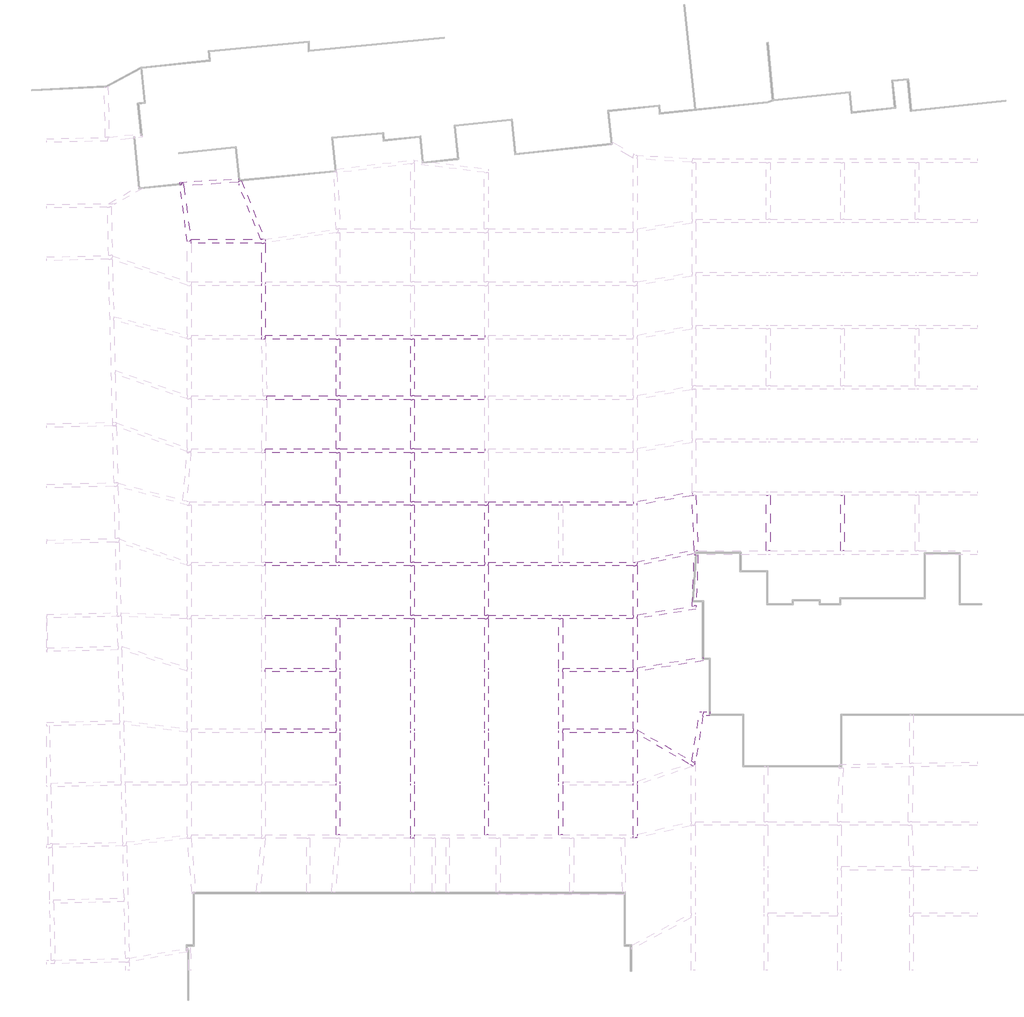
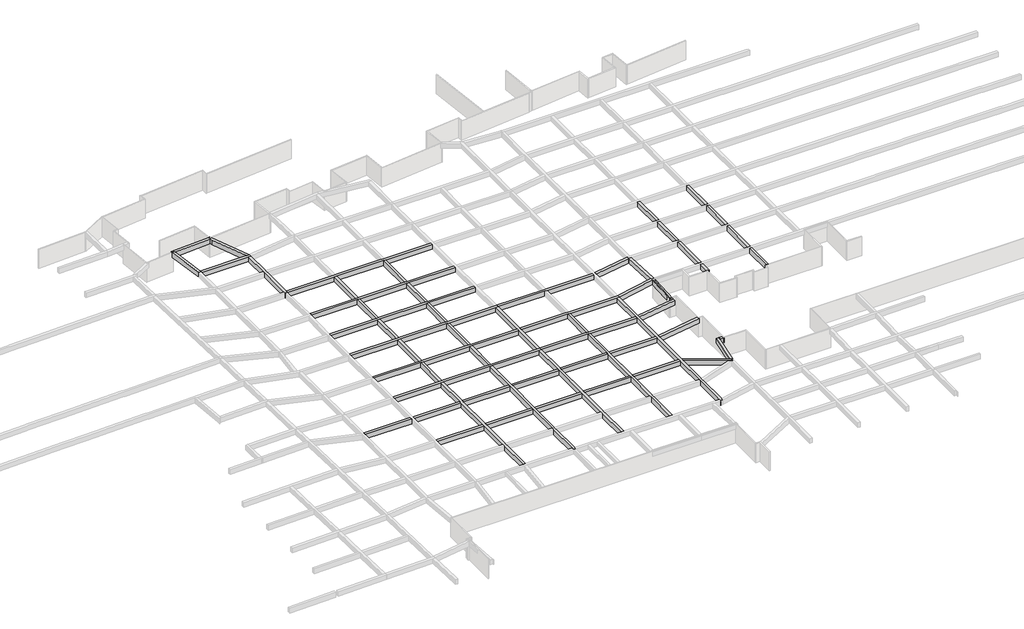
# One storey, part 18 of 20: 44 beams.
"""IFC4 building model written with IfcOpenShell, lengths in millimetres."""

from ifc_helpers import new_model, si_unit, frame, origin, place, context, project, spatial, polyline, outline, extrude, faceted_brep, element, save

model = new_model("IFC4")

# Units and contexts
model_context = context("Model", 3, world=origin())
ifc_project = project(units=[si_unit("LENGTHUNIT", "METRE", prefix="MILLI")], contexts=[model_context])

# Site, building, storey
site = spatial("IfcSite", under=ifc_project)
building = spatial("IfcBuilding", under=site)
storey = spatial("IfcBuildingStorey", under=building, Name="户型图", Elevation=0.0)

# Beams
placement = place(None, origin())
element("IfcBeam", 1, ObjectType="混凝土 - 矩形梁 : KL_beam", at=placement, inside=storey, context=model_context, shape_type="Brep", body=[
    faceted_brep([(54850.0, 183928.0776269, 3300.0), (54825.4500234, 184115.0, 3300.0), (54066.7931438, 189891.3779922, 3300.0), (54031.7451208, 190158.2319997, 3300.0), (53834.3182386, 190137.4815982, 3300.0), (53846.8616542, 190018.1389708, 3300.0), (53649.434772, 189997.3885693, 3300.0), (54450.0, 183901.9223731, 3300.0), (54450.0, 183901.9223731, 2500.0), (53649.434772, 189997.3885693, 2500.0), (54031.7451208, 190158.2319997, 2500.0), (54066.7931438, 189891.3779922, 2500.0), (54825.4500234, 184115.0, 2500.0), (54850.0, 183928.0776269, 2500.0), (53846.8616542, 190018.1389708, 2500.0), (53834.3182386, 190137.4815982, 2500.0)], [[[0, 1, 2, 3, 4, 5, 6, 7]], [[8, 7, 6, 9]], [[10, 11, 12, 13, 8, 9, 14, 15]], [[3, 2, 1, 0, 13, 12, 11, 10]], [[3, 10, 15, 4]], [[5, 14, 9, 6]], [[14, 5, 4, 15]], [[0, 7, 8, 13]]]),
])
element("IfcBeam", 2, ObjectType="混凝土 - 矩形梁 : KL_beam", at=placement, inside=storey, context=model_context, shape_type="Brep", body=[
    faceted_brep([(54825.4500234, 184115.0, 3300.0), (54850.0, 183928.0776269, 3300.0), (54850.0, 183715.0, 3300.0), (62450.0, 183715.0, 3300.0), (62850.0, 183715.0, 3300.0), (62850.0, 183741.1426524, 3300.0), (62850.0, 184115.0, 3300.0), (62636.0146376, 184115.0, 3300.0), (62354.8866617, 184115.0, 3300.0), (62850.0, 183715.0, 2500.0), (54850.0, 183715.0, 2500.0), (62450.0, 183715.0, 2500.0), (54850.0, 183928.0776269, 2500.0), (54825.4500234, 184115.0, 2500.0), (62354.8866617, 184115.0, 2500.0), (62636.0146376, 184115.0, 2500.0), (62850.0, 184115.0, 2500.0), (62850.0, 183741.1426524, 2500.0)], [[[0, 1, 2, 3, 4, 5, 6, 7, 8]], [[9, 4, 3, 2, 10, 11]], [[12, 13, 14, 15, 16, 17, 9, 11, 10]], [[13, 0, 8, 7, 6, 16, 15, 14]], [[1, 0, 13, 12]], [[2, 1, 12, 10]], [[6, 5, 4, 9, 17, 16]]]),
])
element("IfcBeam", 3, ObjectType="混凝土 - 矩形梁 : KL_beam", at=placement, inside=storey, context=model_context, shape_type="Brep", body=[
    faceted_brep([(62450.0, 173390.0, 3300.0), (62454.5621373, 173390.0, 3300.0), (62850.0, 173390.0, 3300.0), (62850.0, 173592.3073852, 3300.0), (62850.0, 173790.0, 3300.0), (62850.0, 179140.0, 3300.0), (62850.0, 179540.0, 3300.0), (62850.0, 183715.0, 3300.0), (62450.0, 183715.0, 3300.0), (62450.0, 179540.0, 3300.0), (62450.0, 179140.0, 3300.0), (62450.0, 173790.0, 3300.0), (62450.0, 173390.0, 2500.0), (62450.0, 183715.0, 2500.0), (62450.0, 179540.0, 2500.0), (62450.0, 179140.0, 2500.0), (62450.0, 173790.0, 2500.0), (62850.0, 173390.0, 2500.0), (62454.5621373, 173390.0, 2500.0), (62850.0, 183715.0, 2500.0), (62850.0, 179540.0, 2500.0), (62850.0, 179140.0, 2500.0), (62850.0, 173790.0, 2500.0), (62850.0, 173592.3073852, 2500.0)], [[[0, 1, 2, 3, 4, 5, 6, 7, 8, 9, 10, 11]], [[12, 0, 11, 10, 9, 8, 13, 14, 15, 16]], [[17, 18, 12, 16, 15, 14, 13, 19, 20, 21, 22, 23]], [[2, 17, 23, 22, 21, 20, 19, 7, 6, 5, 4, 3]], [[8, 7, 19, 13]], [[2, 1, 0, 12, 18, 17]]]),
])
element("IfcBeam", 4, ObjectType="混凝土 - 矩形梁 : KL_beam", at=placement, inside=storey, context=model_context, shape_type="Brep", body=[
    faceted_brep([(86850.0, 155490.0, 3300.0), (86850.0, 155890.0, 3300.0), (86450.0, 155890.0, 3300.0), (78871.1713568, 155890.0, 3300.0), (78471.1713568, 155890.0, 3300.0), (70871.1713568, 155890.0, 3300.0), (70471.1713568, 155890.0, 3300.0), (62850.0, 155890.0, 3300.0), (62850.0, 155490.0, 3300.0), (70471.1713568, 155490.0, 3300.0), (70871.1713568, 155490.0, 3300.0), (78471.1713568, 155490.0, 3300.0), (78871.1713568, 155490.0, 3300.0), (86450.0, 155490.0, 3300.0), (86850.0, 155490.0, 2500.0), (62850.0, 155490.0, 2500.0), (70471.1713568, 155490.0, 2500.0), (70871.1713568, 155490.0, 2500.0), (78471.1713568, 155490.0, 2500.0), (78871.1713568, 155490.0, 2500.0), (86450.0, 155490.0, 2500.0), (86850.0, 155890.0, 2500.0), (62850.0, 155890.0, 2500.0), (70471.1713568, 155890.0, 2500.0), (70871.1713568, 155890.0, 2500.0), (78471.1713568, 155890.0, 2500.0), (78871.1713568, 155890.0, 2500.0), (86450.0, 155890.0, 2500.0)], [[[0, 1, 2, 3, 4, 5, 6, 7, 8, 9, 10, 11, 12, 13]], [[14, 0, 13, 12, 11, 10, 9, 8, 15, 16, 17, 18, 19, 20]], [[21, 14, 20, 19, 18, 17, 16, 15, 22, 23, 24, 25, 26, 27]], [[1, 21, 27, 26, 25, 24, 23, 22, 7, 6, 5, 4, 3, 2]], [[8, 7, 22, 15]], [[1, 0, 14, 21]]]),
])
element("IfcBeam", 5, ObjectType="混凝土 - 矩形梁 : KL_beam", at=placement, inside=storey, context=model_context, shape_type="Brep", body=[
    faceted_brep([(62850.0, 149390.0, 3300.0), (62850.0, 148990.0, 3300.0), (70471.1713568, 148990.0, 3300.0), (70871.1713568, 148990.0, 3300.0), (78471.1713568, 148990.0, 3300.0), (78871.1713568, 148990.0, 3300.0), (86450.0, 148990.0, 3300.0), (86450.0, 149390.0, 3300.0), (78871.1713568, 149390.0, 3300.0), (78471.1713568, 149390.0, 3300.0), (70871.1713568, 149390.0, 3300.0), (70471.1713568, 149390.0, 3300.0), (62850.0, 148990.0, 2500.0), (70471.1713568, 148990.0, 2500.0), (70871.1713568, 148990.0, 2500.0), (78471.1713568, 148990.0, 2500.0), (78871.1713568, 148990.0, 2500.0), (86450.0, 148990.0, 2500.0), (62850.0, 149390.0, 2500.0), (70471.1713568, 149390.0, 2500.0), (70871.1713568, 149390.0, 2500.0), (78471.1713568, 149390.0, 2500.0), (78871.1713568, 149390.0, 2500.0), (86450.0, 149390.0, 2500.0)], [[[0, 1, 2, 3, 4, 5, 6, 7, 8, 9, 10, 11]], [[1, 12, 13, 14, 15, 16, 17, 6, 5, 4, 3, 2]], [[12, 18, 19, 20, 21, 22, 23, 17, 16, 15, 14, 13]], [[18, 0, 11, 10, 9, 8, 7, 23, 22, 21, 20, 19]], [[1, 0, 18, 12]], [[7, 6, 17, 23]]]),
])
element("IfcBeam", 6, ObjectType="混凝土 - 矩形梁 : KL_beam", at=placement, inside=storey, context=model_context, shape_type="Brep", body=[
    faceted_brep([(86850.0, 143290.0, 3300.0), (86850.0, 143690.0, 3300.0), (86450.0, 143690.0, 3300.0), (78871.1713568, 143690.0, 3300.0), (78471.1713568, 143690.0, 3300.0), (70871.1713568, 143690.0, 3300.0), (70471.1713568, 143690.0, 3300.0), (62850.0, 143690.0, 3300.0), (62850.0, 143290.0, 3300.0), (70471.1713568, 143290.0, 3300.0), (70871.1713568, 143290.0, 3300.0), (78471.1713568, 143290.0, 3300.0), (78871.1713568, 143290.0, 3300.0), (86450.0, 143290.0, 3300.0), (86850.0, 143290.0, 2500.0), (62850.0, 143290.0, 2500.0), (70471.1713568, 143290.0, 2500.0), (70871.1713568, 143290.0, 2500.0), (78471.1713568, 143290.0, 2500.0), (78871.1713568, 143290.0, 2500.0), (86450.0, 143290.0, 2500.0), (86850.0, 143690.0, 2500.0), (62850.0, 143690.0, 2500.0), (70471.1713568, 143690.0, 2500.0), (70871.1713568, 143690.0, 2500.0), (78471.1713568, 143690.0, 2500.0), (78871.1713568, 143690.0, 2500.0), (86450.0, 143690.0, 2500.0)], [[[0, 1, 2, 3, 4, 5, 6, 7, 8, 9, 10, 11, 12, 13]], [[14, 0, 13, 12, 11, 10, 9, 8, 15, 16, 17, 18, 19, 20]], [[21, 14, 20, 19, 18, 17, 16, 15, 22, 23, 24, 25, 26, 27]], [[1, 21, 27, 26, 25, 24, 23, 22, 7, 6, 5, 4, 3, 2]], [[8, 7, 22, 15]], [[1, 0, 14, 21]]]),
])
element("IfcBeam", 7, ObjectType="混凝土 - 矩形梁 : KL_beam", at=placement, inside=storey, context=model_context, shape_type="Brep", body=[
    faceted_brep([(62855.332398, 161590.0, 3300.0), (62850.0, 161387.3688765, 3300.0), (62850.0, 161190.0, 3300.0), (70471.1713568, 161190.0, 3300.0), (70871.1713568, 161190.0, 3300.0), (78471.1713568, 161190.0, 3300.0), (78871.1713568, 161190.0, 3300.0), (86450.0, 161190.0, 3300.0), (86450.0, 161590.0, 3300.0), (78871.1713568, 161590.0, 3300.0), (78471.1713568, 161590.0, 3300.0), (70871.1713568, 161590.0, 3300.0), (70471.1713568, 161590.0, 3300.0), (62850.0, 161190.0, 2500.0), (70471.1713568, 161190.0, 2500.0), (70871.1713568, 161190.0, 2500.0), (78471.1713568, 161190.0, 2500.0), (78871.1713568, 161190.0, 2500.0), (86450.0, 161190.0, 2500.0), (62850.0, 161387.3688765, 2500.0), (62855.332398, 161590.0, 2500.0), (70471.1713568, 161590.0, 2500.0), (70871.1713568, 161590.0, 2500.0), (78471.1713568, 161590.0, 2500.0), (78871.1713568, 161590.0, 2500.0), (86450.0, 161590.0, 2500.0)], [[[0, 1, 2, 3, 4, 5, 6, 7, 8, 9, 10, 11, 12]], [[2, 13, 14, 15, 16, 17, 18, 7, 6, 5, 4, 3]], [[19, 20, 21, 22, 23, 24, 25, 18, 17, 16, 15, 14, 13]], [[20, 0, 12, 11, 10, 9, 8, 25, 24, 23, 22, 21]], [[0, 20, 19, 1]], [[2, 1, 19, 13]], [[8, 7, 18, 25]]]),
])
element("IfcBeam", 8, ObjectType="混凝土 - 矩形梁 : KL_beam", at=placement, inside=storey, context=model_context, shape_type="Brep", body=[
    faceted_brep([(63000.0607194, 167089.6762125, 3300.0), (63004.668632, 166890.0, 3300.0), (70471.1713568, 166890.0, 3300.0), (70871.1713568, 166890.0, 3300.0), (78471.1713568, 166890.0, 3300.0), (78871.1713568, 166890.0, 3300.0), (86450.0, 166890.0, 3300.0), (86450.0, 167290.0, 3300.0), (78866.5603873, 167290.0, 3300.0), (78466.5603873, 167290.0, 3300.0), (70871.1713568, 167290.0, 3300.0), (70471.1713568, 167290.0, 3300.0), (63005.332398, 167290.0, 3300.0), (63004.668632, 166890.0, 2500.0), (70471.1713568, 166890.0, 2500.0), (70871.1713568, 166890.0, 2500.0), (78471.1713568, 166890.0, 2500.0), (78871.1713568, 166890.0, 2500.0), (86450.0, 166890.0, 2500.0), (63000.0607194, 167089.6762125, 2500.0), (63005.332398, 167290.0, 2500.0), (70471.1713568, 167290.0, 2500.0), (70871.1713568, 167290.0, 2500.0), (78466.5603873, 167290.0, 2500.0), (78866.5603873, 167290.0, 2500.0), (86450.0, 167290.0, 2500.0)], [[[0, 1, 2, 3, 4, 5, 6, 7, 8, 9, 10, 11, 12]], [[1, 13, 14, 15, 16, 17, 18, 6, 5, 4, 3, 2]], [[13, 19, 20, 21, 22, 23, 24, 25, 18, 17, 16, 15, 14]], [[20, 12, 11, 10, 9, 8, 7, 25, 24, 23, 22, 21]], [[13, 1, 0, 19]], [[0, 12, 20, 19]], [[7, 6, 18, 25]]]),
])
element("IfcBeam", 9, ObjectType="混凝土 - 矩形梁 : KL_beam", at=placement, inside=storey, context=model_context, shape_type="Brep", body=[
    faceted_brep([(62850.0, 173790.0, 3300.0), (62850.0, 173592.3073852, 3300.0), (62854.668632, 173390.0, 3300.0), (70471.1713568, 173390.0, 3300.0), (70871.1713568, 173390.0, 3300.0), (78466.5603873, 173390.0, 3300.0), (78866.5603873, 173390.0, 3300.0), (86450.0, 173390.0, 3300.0), (86450.0, 173790.0, 3300.0), (78866.5603873, 173790.0, 3300.0), (78466.5603873, 173790.0, 3300.0), (70871.1713568, 173790.0, 3300.0), (70471.1713568, 173790.0, 3300.0), (62854.668632, 173390.0, 2500.0), (70471.1713568, 173390.0, 2500.0), (70871.1713568, 173390.0, 2500.0), (78466.5603873, 173390.0, 2500.0), (78866.5603873, 173390.0, 2500.0), (86450.0, 173390.0, 2500.0), (62850.0, 173592.3073852, 2500.0), (62850.0, 173790.0, 2500.0), (70471.1713568, 173790.0, 2500.0), (70871.1713568, 173790.0, 2500.0), (78466.5603873, 173790.0, 2500.0), (78866.5603873, 173790.0, 2500.0), (86450.0, 173790.0, 2500.0)], [[[0, 1, 2, 3, 4, 5, 6, 7, 8, 9, 10, 11, 12]], [[2, 13, 14, 15, 16, 17, 18, 7, 6, 5, 4, 3]], [[19, 20, 21, 22, 23, 24, 25, 18, 17, 16, 15, 14, 13]], [[20, 0, 12, 11, 10, 9, 8, 25, 24, 23, 22, 21]], [[0, 20, 19, 1]], [[2, 1, 19, 13]], [[8, 7, 18, 25]]]),
])
element("IfcBeam", 10, ObjectType="混凝土 - 矩形梁 : KL_beam", at=placement, inside=storey, context=model_context, shape_type="Brep", body=[
    faceted_brep([(60034.1132037, 189932.4884269, 3300.0), (60034.1132037, 189932.4884269, 2500.0), (62354.8866617, 184115.0, 2500.0), (62354.8866617, 184115.0, 3300.0), (59999.9831265, 190257.2144199, 3300.0), (59985.5481909, 190394.5536585, 3300.0), (59985.5481909, 190394.5536585, 2500.0), (59999.9831265, 190257.2144199, 2500.0), (60269.4868427, 190421.9993923, 3300.0), (60269.4868427, 190421.9993923, 2500.0), (62450.0, 184115.0, 2500.0), (62636.0146376, 184115.0, 2500.0), (62636.0146376, 184115.0, 3300.0), (62450.0, 184115.0, 3300.0), (62777.6028574, 184134.8989266, 3300.0), (62777.6028574, 184134.8989266, 2500.0)], [[[0, 1, 2, 3]], [[1, 0, 4, 5, 6, 7]], [[5, 8, 9, 6]], [[3, 2, 10, 11, 12, 13]], [[5, 4, 0, 3, 13, 12, 14, 8]], [[1, 7, 6, 9, 15, 11, 10, 2]], [[9, 8, 14, 15]], [[12, 11, 15, 14]]]),
])
element("IfcBeam", 11, ObjectType="混凝土 - 矩形梁 : KL_beam", at=placement, inside=storey, context=model_context, shape_type="Brep", body=[
    faceted_brep([(60171.1392883, 190668.5274444, 3300.0), (60078.0168735, 190662.7855801, 3300.0), (60092.4518091, 190525.4463415, 3300.0), (60223.1777857, 190538.0824174, 3300.0), (60078.0168735, 190662.7855801, 2500.0), (60171.1392883, 190668.5274444, 2500.0), (60223.1777857, 190538.0824174, 2500.0), (60092.4518091, 190525.4463415, 2500.0)], [[[0, 1, 2, 3]], [[4, 5, 6, 7]], [[0, 5, 4, 1]], [[5, 0, 3, 6]], [[2, 1, 4, 7]], [[3, 2, 7, 6]]]),
    faceted_brep([(59999.9831265, 190257.2144199, 2500.0), (59999.9831265, 190257.2144199, 3300.0), (54066.7931438, 189891.3779922, 3300.0), (54066.7931438, 189891.3779922, 2500.0), (53614.386749, 190264.2425768, 3300.0), (53614.386749, 190264.2425768, 2500.0), (53633.8032011, 190116.4066185, 2500.0), (53633.8032011, 190116.4066185, 3300.0), (59958.1328072, 190655.3936108, 2500.0), (59958.1328072, 190655.3936108, 3300.0), (59985.5481909, 190394.5536585, 3300.0), (59985.5481909, 190394.5536585, 2500.0), (53834.3182386, 190137.4815982, 2500.0), (54031.7451208, 190158.2319997, 2500.0), (54031.7451208, 190158.2319997, 3300.0), (53834.3182386, 190137.4815982, 3300.0)], [[[0, 1, 2, 3]], [[4, 5, 6, 7]], [[8, 9, 10, 1, 0, 11]], [[5, 4, 9, 8]], [[7, 6, 12, 13, 14, 15]], [[9, 4, 7, 15, 14, 2, 1, 10]], [[5, 8, 11, 0, 3, 13, 12, 6]], [[14, 13, 3, 2]]]),
])
element("IfcBeam", 12, ObjectType="混凝土 - 矩形梁 : KL_beam", at=placement, inside=storey, context=model_context, shape_type="SweptSolid", body=[
    extrude(outline(polyline([(70871.1713568, 167290.0), (70471.1713568, 167290.0), (70471.1713568, 173390.0), (70871.1713568, 173390.0), (70871.1713568, 167290.0)])), frame((0.0, 0.0, 2500.0), z_axis=(0.0, 0.0, 1.0), x_axis=(1.0, 0.0, 0.0)), (0.0, 0.0, 1.0), 800.0),
])
element("IfcBeam", 13, ObjectType="混凝土 - 矩形梁 : KL_beam", at=placement, inside=storey, context=model_context, shape_type="SweptSolid", body=[
    extrude(outline(polyline([(70871.1713568, 161590.0), (70471.1713568, 161590.0), (70471.1713568, 166890.0), (70871.1713568, 166890.0), (70871.1713568, 161590.0)])), frame((0.0, 0.0, 2500.0), z_axis=(0.0, 0.0, 1.0), x_axis=(1.0, 0.0, 0.0)), (0.0, 0.0, 1.0), 800.0),
])
element("IfcBeam", 14, ObjectType="混凝土 - 矩形梁 : KL_beam", at=placement, inside=storey, context=model_context, shape_type="SweptSolid", body=[
    extrude(outline(polyline([(70871.1713568, 155890.0), (70471.1713568, 155890.0), (70471.1713568, 161190.0), (70871.1713568, 161190.0), (70871.1713568, 155890.0)])), frame((0.0, 0.0, 2500.0), z_axis=(0.0, 0.0, 1.0), x_axis=(1.0, 0.0, 0.0)), (0.0, 0.0, 1.0), 800.0),
])
element("IfcBeam", 15, ObjectType="混凝土 - 矩形梁 : KL_beam", at=placement, inside=storey, context=model_context, shape_type="SweptSolid", body=[
    extrude(outline(polyline([(70471.1713568, 155490.0), (70871.1713568, 155490.0), (70871.1713568, 149390.0), (70471.1713568, 149390.0), (70471.1713568, 155490.0)])), frame((0.0, 0.0, 2500.0), z_axis=(0.0, 0.0, 1.0), x_axis=(1.0, 0.0, 0.0)), (0.0, 0.0, 1.0), 800.0),
    extrude(outline(polyline([(70871.1713568, 143690.0), (70471.1713568, 143690.0), (70471.1713568, 148990.0), (70871.1713568, 148990.0), (70871.1713568, 143690.0)])), frame((0.0, 0.0, 2500.0), z_axis=(0.0, 0.0, 1.0), x_axis=(1.0, 0.0, 0.0)), (0.0, 0.0, 1.0), 800.0),
])
element("IfcBeam", 16, ObjectType="混凝土 - 矩形梁 : KL_beam", at=placement, inside=storey, context=model_context, shape_type="SweptSolid", body=[
    extrude(outline(polyline([(78471.1713568, 148990.0), (78871.1713568, 148990.0), (78871.1713568, 143690.0), (78471.1713568, 143690.0), (78471.1713568, 148990.0)])), frame((0.0, 0.0, 2500.0), z_axis=(0.0, 0.0, 1.0), x_axis=(1.0, 0.0, 0.0)), (0.0, 0.0, 1.0), 800.0),
])
element("IfcBeam", 17, ObjectType="混凝土 - 矩形梁 : KL_beam", at=placement, inside=storey, context=model_context, shape_type="SweptSolid", body=[
    extrude(outline(polyline([(78471.1713568, 155490.0), (78871.1713568, 155490.0), (78871.1713568, 149390.0), (78471.1713568, 149390.0), (78471.1713568, 155490.0)])), frame((0.0, 0.0, 2500.0), z_axis=(0.0, 0.0, 1.0), x_axis=(1.0, 0.0, 0.0)), (0.0, 0.0, 1.0), 800.0),
])
element("IfcBeam", 18, ObjectType="混凝土 - 矩形梁 : KL_beam", at=placement, inside=storey, context=model_context, shape_type="SweptSolid", body=[
    extrude(outline(polyline([(78871.1713568, 155890.0), (78471.1713568, 155890.0), (78471.1713568, 161190.0), (78871.1713568, 161190.0), (78871.1713568, 155890.0)])), frame((0.0, 0.0, 2500.0), z_axis=(0.0, 0.0, 1.0), x_axis=(1.0, 0.0, 0.0)), (0.0, 0.0, 1.0), 800.0),
])
element("IfcBeam", 19, ObjectType="混凝土 - 矩形梁 : KL_beam", at=placement, inside=storey, context=model_context, shape_type="SweptSolid", body=[
    extrude(outline(polyline([(78871.1713568, 161590.0), (78471.1713568, 161590.0), (78471.1713568, 166890.0), (78871.1713568, 166890.0), (78871.1713568, 161590.0)])), frame((0.0, 0.0, 2500.0), z_axis=(0.0, 0.0, 1.0), x_axis=(1.0, 0.0, 0.0)), (0.0, 0.0, 1.0), 800.0),
])
element("IfcBeam", 20, ObjectType="混凝土 - 矩形梁 : KL_beam", at=placement, inside=storey, context=model_context, shape_type="SweptSolid", body=[
    extrude(outline(polyline([(78866.5603873, 167290.0), (78466.5603873, 167290.0), (78466.5603873, 173390.0), (78866.5603873, 173390.0), (78866.5603873, 167290.0)])), frame((0.0, 0.0, 2500.0), z_axis=(0.0, 0.0, 1.0), x_axis=(1.0, 0.0, 0.0)), (0.0, 0.0, 1.0), 800.0),
])
element("IfcBeam", 21, ObjectType="混凝土 - 矩形梁 : KL_beam", at=placement, inside=storey, context=model_context, shape_type="Brep", body=[
    faceted_brep([(86850.0, 155490.0, 3300.0), (86450.0, 155490.0, 3300.0), (86450.0, 149390.0, 3300.0), (86450.0, 148990.0, 3300.0), (86450.0, 143690.0, 3300.0), (86850.0, 143690.0, 3300.0), (86850.0, 148990.0, 3300.0), (86850.0, 149390.0, 3300.0), (86450.0, 155490.0, 2500.0), (86450.0, 149390.0, 2500.0), (86450.0, 148990.0, 2500.0), (86450.0, 143690.0, 2500.0), (86850.0, 155490.0, 2500.0), (86850.0, 149390.0, 2500.0), (86850.0, 148990.0, 2500.0), (86850.0, 143690.0, 2500.0)], [[[0, 1, 2, 3, 4, 5, 6, 7]], [[1, 8, 9, 10, 11, 4, 3, 2]], [[8, 12, 13, 14, 15, 11, 10, 9]], [[12, 0, 7, 6, 5, 15, 14, 13]], [[1, 0, 12, 8]], [[5, 4, 11, 15]]]),
])
element("IfcBeam", 22, ObjectType="混凝土 - 矩形梁 : KL_beam", at=placement, inside=storey, context=model_context, shape_type="Brep", body=[
    faceted_brep([(86850.0, 155890.0, 3300.0), (86850.0, 155490.0, 3300.0), (94423.4648002, 155490.0, 3300.0), (94823.4648002, 155490.0, 3300.0), (102450.0, 155490.0, 3300.0), (102450.0, 155890.0, 3300.0), (94823.4648002, 155890.0, 3300.0), (94423.4648002, 155890.0, 3300.0), (86850.0, 155490.0, 2500.0), (94423.4648002, 155490.0, 2500.0), (94823.4648002, 155490.0, 2500.0), (102450.0, 155490.0, 2500.0), (86850.0, 155890.0, 2500.0), (94423.4648002, 155890.0, 2500.0), (94823.4648002, 155890.0, 2500.0), (102450.0, 155890.0, 2500.0)], [[[0, 1, 2, 3, 4, 5, 6, 7]], [[1, 8, 9, 10, 11, 4, 3, 2]], [[8, 12, 13, 14, 15, 11, 10, 9]], [[12, 0, 7, 6, 5, 15, 14, 13]], [[1, 0, 12, 8]], [[5, 4, 11, 15]]]),
])
element("IfcBeam", 23, ObjectType="混凝土 - 矩形梁 : KL_beam", at=placement, inside=storey, context=model_context, shape_type="Brep", body=[
    faceted_brep([(102850.0, 148990.0, 3300.0), (102850.0, 149026.9931985, 3300.0), (102850.0, 149390.0, 3300.0), (102450.0, 149390.0, 3300.0), (94823.4648002, 149390.0, 3300.0), (94423.4648002, 149390.0, 3300.0), (86850.0, 149390.0, 3300.0), (86850.0, 148990.0, 3300.0), (94423.4648002, 148990.0, 3300.0), (94823.4648002, 148990.0, 3300.0), (102450.0, 148990.0, 3300.0), (102850.0, 148990.0, 2500.0), (86850.0, 148990.0, 2500.0), (94423.4648002, 148990.0, 2500.0), (94823.4648002, 148990.0, 2500.0), (102450.0, 148990.0, 2500.0), (102850.0, 149390.0, 2500.0), (102850.0, 149026.9931985, 2500.0), (86850.0, 149390.0, 2500.0), (94423.4648002, 149390.0, 2500.0), (94823.4648002, 149390.0, 2500.0), (102450.0, 149390.0, 2500.0)], [[[0, 1, 2, 3, 4, 5, 6, 7, 8, 9, 10]], [[11, 0, 10, 9, 8, 7, 12, 13, 14, 15]], [[16, 17, 11, 15, 14, 13, 12, 18, 19, 20, 21]], [[2, 16, 21, 20, 19, 18, 6, 5, 4, 3]], [[7, 6, 18, 12]], [[2, 1, 0, 11, 17, 16]]]),
])
element("IfcBeam", 24, ObjectType="混凝土 - 矩形梁 : KL_beam", at=placement, inside=storey, context=model_context, shape_type="Brep", body=[
    faceted_brep([(86850.0, 143690.0, 3300.0), (86850.0, 143290.0, 3300.0), (94423.4648002, 143290.0, 3300.0), (94823.4648002, 143290.0, 3300.0), (102450.0, 143290.0, 3300.0), (102450.0, 143690.0, 3300.0), (94823.4648002, 143690.0, 3300.0), (94423.4648002, 143690.0, 3300.0), (86850.0, 143290.0, 2500.0), (94423.4648002, 143290.0, 2500.0), (94823.4648002, 143290.0, 2500.0), (102450.0, 143290.0, 2500.0), (86850.0, 143690.0, 2500.0), (94423.4648002, 143690.0, 2500.0), (94823.4648002, 143690.0, 2500.0), (102450.0, 143690.0, 2500.0)], [[[0, 1, 2, 3, 4, 5, 6, 7]], [[1, 8, 9, 10, 11, 4, 3, 2]], [[8, 12, 13, 14, 15, 11, 10, 9]], [[12, 0, 7, 6, 5, 15, 14, 13]], [[1, 0, 12, 8]], [[5, 4, 11, 15]]]),
])
element("IfcBeam", 25, ObjectType="混凝土 - 矩形梁 : KL_beam", at=placement, inside=storey, context=model_context, shape_type="Brep", body=[
    faceted_brep([(102850.0, 119729.9007984, 3300.0), (102850.0, 120139.8450935, 3300.0), (102850.0, 125421.4252388, 3300.0), (102850.0, 125843.4152433, 3300.0), (102850.0, 130914.5836602, 3300.0), (102850.0, 131376.4638755, 3300.0), (102850.0, 137632.1126937, 3300.0), (102850.0, 138037.3913563, 3300.0), (102850.0, 143319.1838629, 3300.0), (102850.0, 143724.1699132, 3300.0), (102850.0, 148990.0, 3300.0), (102450.0, 148990.0, 3300.0), (102450.0, 143690.0, 3300.0), (102450.0, 143290.0, 3300.0), (102450.0, 138002.152967, 3300.0), (102450.0, 137602.152967, 3300.0), (102450.0, 131460.9938217, 3300.0), (102450.0, 131060.9938217, 3300.0), (102450.0, 125765.1975441, 3300.0), (102450.0, 125365.1975441, 3300.0), (102450.0, 120090.0, 3300.0), (102450.0, 119729.9007984, 3300.0), (102450.0, 148990.0, 2500.0), (102450.0, 143690.0, 2500.0), (102450.0, 143290.0, 2500.0), (102450.0, 138002.152967, 2500.0), (102450.0, 137602.152967, 2500.0), (102450.0, 131460.9938217, 2500.0), (102450.0, 131060.9938217, 2500.0), (102450.0, 125765.1975441, 2500.0), (102450.0, 125365.1975441, 2500.0), (102450.0, 120090.0, 2500.0), (102450.0, 119729.9007984, 2500.0), (102850.0, 148990.0, 2500.0), (102850.0, 143724.1699132, 2500.0), (102850.0, 143319.1838629, 2500.0), (102850.0, 138037.3913563, 2500.0), (102850.0, 137632.1126937, 2500.0), (102850.0, 131376.4638755, 2500.0), (102850.0, 130914.5836602, 2500.0), (102850.0, 125843.4152433, 2500.0), (102850.0, 125421.4252388, 2500.0), (102850.0, 120139.8450935, 2500.0), (102850.0, 119729.9007984, 2500.0)], [[[0, 1, 2, 3, 4, 5, 6, 7, 8, 9, 10, 11, 12, 13, 14, 15, 16, 17, 18, 19, 20, 21]], [[21, 20, 19, 18, 17, 16, 15, 14, 13, 12, 11, 22, 23, 24, 25, 26, 27, 28, 29, 30, 31, 32]], [[32, 31, 30, 29, 28, 27, 26, 25, 24, 23, 22, 33, 34, 35, 36, 37, 38, 39, 40, 41, 42, 43]], [[10, 9, 8, 7, 6, 5, 4, 3, 2, 1, 0, 43, 42, 41, 40, 39, 38, 37, 36, 35, 34, 33]], [[11, 10, 33, 22]], [[0, 21, 32, 43]]]),
])
element("IfcBeam", 26, ObjectType="混凝土 - 矩形梁 : KL_beam", at=placement, inside=storey, context=model_context, shape_type="Brep", body=[
    faceted_brep([(94823.4648002, 148990.0, 3300.0), (94423.4648002, 148990.0, 3300.0), (94423.4648002, 143690.0, 3300.0), (94823.4648002, 143690.0, 3300.0), (94423.4648002, 148990.0, 2500.0), (94423.4648002, 143690.0, 2500.0), (94823.4648002, 148990.0, 2500.0), (94823.4648002, 143690.0, 2500.0)], [[[0, 1, 2, 3]], [[1, 4, 5, 2]], [[4, 6, 7, 5]], [[6, 0, 3, 7]], [[1, 0, 6, 4]], [[3, 2, 5, 7]]]),
    faceted_brep([(94423.4648002, 143290.0, 3300.0), (94823.4648002, 143290.0, 3300.0), (94823.4648002, 143290.0, 2500.0), (94423.4648002, 143290.0, 2500.0), (94423.4648002, 138002.152967, 3300.0), (94423.4648002, 137602.152967, 3300.0), (94423.4648002, 131460.9938217, 3300.0), (94423.4648002, 131060.9938217, 3300.0), (94423.4648002, 125765.1975441, 3300.0), (94423.4648002, 125365.1975441, 3300.0), (94423.4648002, 120090.0, 3300.0), (94823.4648002, 120090.0, 3300.0), (94823.4648002, 125365.1975441, 3300.0), (94823.4648002, 125765.1975441, 3300.0), (94823.4648002, 131060.9938217, 3300.0), (94823.4648002, 131460.9938217, 3300.0), (94823.4648002, 137602.152967, 3300.0), (94823.4648002, 138002.152967, 3300.0), (94423.4648002, 138002.152967, 2500.0), (94423.4648002, 137602.152967, 2500.0), (94423.4648002, 131460.9938217, 2500.0), (94423.4648002, 131060.9938217, 2500.0), (94423.4648002, 125765.1975441, 2500.0), (94423.4648002, 125365.1975441, 2500.0), (94423.4648002, 120090.0, 2500.0), (94823.4648002, 138002.152967, 2500.0), (94823.4648002, 137602.152967, 2500.0), (94823.4648002, 131460.9938217, 2500.0), (94823.4648002, 131060.9938217, 2500.0), (94823.4648002, 125765.1975441, 2500.0), (94823.4648002, 125365.1975441, 2500.0), (94823.4648002, 120090.0, 2500.0)], [[[0, 1, 2, 3]], [[1, 0, 4, 5, 6, 7, 8, 9, 10, 11, 12, 13, 14, 15, 16, 17]], [[0, 3, 18, 19, 20, 21, 22, 23, 24, 10, 9, 8, 7, 6, 5, 4]], [[3, 2, 25, 26, 27, 28, 29, 30, 31, 24, 23, 22, 21, 20, 19, 18]], [[2, 1, 17, 16, 15, 14, 13, 12, 11, 31, 30, 29, 28, 27, 26, 25]], [[11, 10, 24, 31]]]),
])
element("IfcBeam", 27, ObjectType="混凝土 - 矩形梁 : KL_beam", at=placement, inside=storey, context=model_context, shape_type="Brep", body=[
    faceted_brep([(86850.0, 143290.0, 3300.0), (86450.0, 143290.0, 3300.0), (86450.0, 138002.152967, 3300.0), (86450.0, 137602.152967, 3300.0), (86450.0, 131460.9938217, 3300.0), (86450.0, 131060.9938217, 3300.0), (86450.0, 125765.1975441, 3300.0), (86450.0, 125365.1975441, 3300.0), (86450.0, 120090.0, 3300.0), (86850.0, 120090.0, 3300.0), (86850.0, 125365.1975441, 3300.0), (86850.0, 125765.1975441, 3300.0), (86850.0, 131060.9938217, 3300.0), (86850.0, 131460.9938217, 3300.0), (86850.0, 137602.152967, 3300.0), (86850.0, 138002.152967, 3300.0), (86450.0, 143290.0, 2500.0), (86450.0, 138002.152967, 2500.0), (86450.0, 137602.152967, 2500.0), (86450.0, 131460.9938217, 2500.0), (86450.0, 131060.9938217, 2500.0), (86450.0, 125765.1975441, 2500.0), (86450.0, 125365.1975441, 2500.0), (86450.0, 120090.0, 2500.0), (86850.0, 143290.0, 2500.0), (86850.0, 138002.152967, 2500.0), (86850.0, 137602.152967, 2500.0), (86850.0, 131460.9938217, 2500.0), (86850.0, 131060.9938217, 2500.0), (86850.0, 125765.1975441, 2500.0), (86850.0, 125365.1975441, 2500.0), (86850.0, 120090.0, 2500.0)], [[[0, 1, 2, 3, 4, 5, 6, 7, 8, 9, 10, 11, 12, 13, 14, 15]], [[1, 16, 17, 18, 19, 20, 21, 22, 23, 8, 7, 6, 5, 4, 3, 2]], [[16, 24, 25, 26, 27, 28, 29, 30, 31, 23, 22, 21, 20, 19, 18, 17]], [[24, 0, 15, 14, 13, 12, 11, 10, 9, 31, 30, 29, 28, 27, 26, 25]], [[1, 0, 24, 16]], [[9, 8, 23, 31]]]),
])
element("IfcBeam", 28, ObjectType="混凝土 - 矩形梁 : KL_beam", at=placement, inside=storey, context=model_context, shape_type="Brep", body=[
    faceted_brep([(78471.1713568, 119690.0, 3300.0), (78871.1713568, 119690.0, 3300.0), (78871.1713568, 120090.0, 3300.0), (78871.1713568, 125365.1975441, 3300.0), (78871.1713568, 125765.1975441, 3300.0), (78871.1713568, 131060.9938217, 3300.0), (78871.1713568, 131460.9938217, 3300.0), (78871.1713568, 137602.152967, 3300.0), (78871.1713568, 138002.152967, 3300.0), (78871.1713568, 143290.0, 3300.0), (78471.1713568, 143290.0, 3300.0), (78471.1713568, 138002.152967, 3300.0), (78471.1713568, 137602.152967, 3300.0), (78471.1713568, 131460.9938217, 3300.0), (78471.1713568, 131060.9938217, 3300.0), (78471.1713568, 125765.1975441, 3300.0), (78471.1713568, 125365.1975441, 3300.0), (78471.1713568, 120090.0, 3300.0), (78471.1713568, 119690.0, 2500.0), (78471.1713568, 143290.0, 2500.0), (78471.1713568, 138002.152967, 2500.0), (78471.1713568, 137602.152967, 2500.0), (78471.1713568, 131460.9938217, 2500.0), (78471.1713568, 131060.9938217, 2500.0), (78471.1713568, 125765.1975441, 2500.0), (78471.1713568, 125365.1975441, 2500.0), (78471.1713568, 120090.0, 2500.0), (78871.1713568, 119690.0, 2500.0), (78871.1713568, 143290.0, 2500.0), (78871.1713568, 138002.152967, 2500.0), (78871.1713568, 137602.152967, 2500.0), (78871.1713568, 131460.9938217, 2500.0), (78871.1713568, 131060.9938217, 2500.0), (78871.1713568, 125765.1975441, 2500.0), (78871.1713568, 125365.1975441, 2500.0), (78871.1713568, 120090.0, 2500.0)], [[[0, 1, 2, 3, 4, 5, 6, 7, 8, 9, 10, 11, 12, 13, 14, 15, 16, 17]], [[18, 0, 17, 16, 15, 14, 13, 12, 11, 10, 19, 20, 21, 22, 23, 24, 25, 26]], [[27, 18, 26, 25, 24, 23, 22, 21, 20, 19, 28, 29, 30, 31, 32, 33, 34, 35]], [[1, 27, 35, 34, 33, 32, 31, 30, 29, 28, 9, 8, 7, 6, 5, 4, 3, 2]], [[10, 9, 28, 19]], [[1, 0, 18, 27]]]),
])
element("IfcBeam", 29, ObjectType="混凝土 - 矩形梁 : KL_beam", at=placement, inside=storey, context=model_context, shape_type="Brep", body=[
    faceted_brep([(70871.1713568, 143290.0, 3300.0), (70471.1713568, 143290.0, 3300.0), (70471.1713568, 138002.152967, 3300.0), (70471.1713568, 137602.152967, 3300.0), (70471.1713568, 131460.9938217, 3300.0), (70471.1713568, 131060.9938217, 3300.0), (70471.1713568, 125765.1975441, 3300.0), (70471.1713568, 125365.1975441, 3300.0), (70471.1713568, 120090.0, 3300.0), (70871.1713568, 120090.0, 3300.0), (70871.1713568, 125365.1975441, 3300.0), (70871.1713568, 125765.1975441, 3300.0), (70871.1713568, 131060.9938217, 3300.0), (70871.1713568, 131460.9938217, 3300.0), (70871.1713568, 137602.152967, 3300.0), (70871.1713568, 138002.152967, 3300.0), (70471.1713568, 143290.0, 2500.0), (70471.1713568, 138002.152967, 2500.0), (70471.1713568, 137602.152967, 2500.0), (70471.1713568, 131460.9938217, 2500.0), (70471.1713568, 131060.9938217, 2500.0), (70471.1713568, 125765.1975441, 2500.0), (70471.1713568, 125365.1975441, 2500.0), (70471.1713568, 120090.0, 2500.0), (70871.1713568, 143290.0, 2500.0), (70871.1713568, 138002.152967, 2500.0), (70871.1713568, 137602.152967, 2500.0), (70871.1713568, 131460.9938217, 2500.0), (70871.1713568, 131060.9938217, 2500.0), (70871.1713568, 125765.1975441, 2500.0), (70871.1713568, 125365.1975441, 2500.0), (70871.1713568, 120090.0, 2500.0)], [[[0, 1, 2, 3, 4, 5, 6, 7, 8, 9, 10, 11, 12, 13, 14, 15]], [[1, 16, 17, 18, 19, 20, 21, 22, 23, 8, 7, 6, 5, 4, 3, 2]], [[16, 24, 25, 26, 27, 28, 29, 30, 31, 23, 22, 21, 20, 19, 18, 17]], [[24, 0, 15, 14, 13, 12, 11, 10, 9, 31, 30, 29, 28, 27, 26, 25]], [[1, 0, 24, 16]], [[9, 8, 23, 31]]]),
])
element("IfcBeam", 30, ObjectType="混凝土 - 矩形梁 : KL_beam", at=placement, inside=storey, context=model_context, shape_type="SweptSolid", body=[
    extrude(outline(polyline([(62850.0, 131060.9938217), (62850.0, 131460.9938217), (70471.1713568, 131460.9938217), (70471.1713568, 131060.9938217), (62850.0, 131060.9938217)])), frame((0.0, 0.0, 2500.0), z_axis=(0.0, 0.0, 1.0), x_axis=(1.0, 0.0, 0.0)), (0.0, 0.0, 1.0), 800.0),
    extrude(outline(polyline([(78471.1713568, 131460.9938217), (78471.1713568, 131060.9938217), (70871.1713568, 131060.9938217), (70871.1713568, 131460.9938217), (78471.1713568, 131460.9938217)])), frame((0.0, 0.0, 2500.0), z_axis=(0.0, 0.0, 1.0), x_axis=(1.0, 0.0, 0.0)), (0.0, 0.0, 1.0), 800.0),
])
element("IfcBeam", 31, ObjectType="混凝土 - 矩形梁 : KL_beam", at=placement, inside=storey, context=model_context, shape_type="SweptSolid", body=[
    extrude(outline(polyline([(54850.0, 137602.152967), (54850.0, 138002.152967), (62450.0, 138002.152967), (62450.0, 137602.152967), (54850.0, 137602.152967)])), frame((0.0, 0.0, 2500.0), z_axis=(0.0, 0.0, 1.0), x_axis=(1.0, 0.0, 0.0)), (0.0, 0.0, 1.0), 800.0),
    extrude(outline(polyline([(78471.1713568, 138002.152967), (78471.1713568, 137602.152967), (70871.1713568, 137602.152967), (70871.1713568, 138002.152967), (78471.1713568, 138002.152967)])), frame((0.0, 0.0, 2500.0), z_axis=(0.0, 0.0, 1.0), x_axis=(1.0, 0.0, 0.0)), (0.0, 0.0, 1.0), 800.0),
    extrude(outline(polyline([(70471.1713568, 138002.152967), (70471.1713568, 137602.152967), (62850.0, 137602.152967), (62850.0, 138002.152967), (70471.1713568, 138002.152967)])), frame((0.0, 0.0, 2500.0), z_axis=(0.0, 0.0, 1.0), x_axis=(1.0, 0.0, 0.0)), (0.0, 0.0, 1.0), 800.0),
])
element("IfcBeam", 32, ObjectType="混凝土 - 矩形梁 : KL_beam", at=placement, inside=storey, context=model_context, shape_type="SweptSolid", body=[
    extrude(outline(polyline([(78871.1713568, 137602.152967), (78871.1713568, 138002.152967), (86450.0, 138002.152967), (86450.0, 137602.152967), (78871.1713568, 137602.152967)])), frame((0.0, 0.0, 2500.0), z_axis=(0.0, 0.0, 1.0), x_axis=(1.0, 0.0, 0.0)), (0.0, 0.0, 1.0), 800.0),
    extrude(outline(polyline([(102450.0, 138002.152967), (102450.0, 137602.152967), (94823.4648002, 137602.152967), (94823.4648002, 138002.152967), (102450.0, 138002.152967)])), frame((0.0, 0.0, 2500.0), z_axis=(0.0, 0.0, 1.0), x_axis=(1.0, 0.0, 0.0)), (0.0, 0.0, 1.0), 800.0),
    extrude(outline(polyline([(94423.4648002, 138002.152967), (94423.4648002, 137602.152967), (86850.0, 137602.152967), (86850.0, 138002.152967), (94423.4648002, 138002.152967)])), frame((0.0, 0.0, 2500.0), z_axis=(0.0, 0.0, 1.0), x_axis=(1.0, 0.0, 0.0)), (0.0, 0.0, 1.0), 800.0),
])
element("IfcBeam", 33, ObjectType="混凝土 - 矩形梁 : KL_beam", at=placement, inside=storey, context=model_context, shape_type="SweptSolid", body=[
    extrude(outline(polyline([(78871.1713568, 131060.9938217), (78871.1713568, 131460.9938217), (86450.0, 131460.9938217), (86450.0, 131060.9938217), (78871.1713568, 131060.9938217)])), frame((0.0, 0.0, 2500.0), z_axis=(0.0, 0.0, 1.0), x_axis=(1.0, 0.0, 0.0)), (0.0, 0.0, 1.0), 800.0),
    extrude(outline(polyline([(102450.0, 131460.9938217), (102450.0, 131060.9938217), (94823.4648002, 131060.9938217), (94823.4648002, 131460.9938217), (102450.0, 131460.9938217)])), frame((0.0, 0.0, 2500.0), z_axis=(0.0, 0.0, 1.0), x_axis=(1.0, 0.0, 0.0)), (0.0, 0.0, 1.0), 800.0),
    extrude(outline(polyline([(94423.4648002, 131460.9938217), (94423.4648002, 131060.9938217), (86850.0, 131060.9938217), (86850.0, 131460.9938217), (94423.4648002, 131460.9938217)])), frame((0.0, 0.0, 2500.0), z_axis=(0.0, 0.0, 1.0), x_axis=(1.0, 0.0, 0.0)), (0.0, 0.0, 1.0), 800.0),
])
element("IfcBeam", 34, ObjectType="混凝土 - 矩形梁 : KL_beam", at=placement, inside=storey, context=model_context, shape_type="Brep", body=[
    faceted_brep([(108863.5483185, 127442.6599197, 3300.0), (109063.5483185, 127789.0700812, 3300.0), (108907.217496, 127879.3277237, 3300.0), (108733.3679509, 127979.6998053, 3300.0), (102850.0, 131376.4638755, 3300.0), (102850.0, 130914.5836602, 3300.0), (108401.581434, 127709.3766248, 3300.0), (108863.5483185, 127442.6599197, 2500.0), (102850.0, 130914.5836602, 2500.0), (108401.581434, 127709.3766248, 2500.0), (109063.5483185, 127789.0700812, 2500.0), (102850.0, 131376.4638755, 2500.0), (108733.3679509, 127979.6998053, 2500.0), (108907.217496, 127879.3277237, 2500.0)], [[[0, 1, 2, 3, 4, 5, 6]], [[7, 0, 6, 5, 8, 9]], [[10, 7, 9, 8, 11, 12, 13]], [[1, 10, 13, 12, 11, 4, 3, 2]], [[5, 4, 11, 8]], [[1, 0, 7, 10]]]),
])
element("IfcBeam", 35, ObjectType="混凝土 - 矩形梁 : KL_beam", at=placement, inside=storey, context=model_context, shape_type="Brep", body=[
    faceted_brep([(109157.9751895, 156589.0, 3300.0), (109150.0, 156589.0, 3300.0), (108757.6693662, 156589.0, 3300.0), (108759.0900274, 156552.6765347, 3300.0), (108988.014361, 150699.5391734, 3300.0), (108992.0248105, 150597.0, 3300.0), (109392.3306338, 150597.0, 3300.0), (108757.6693662, 156589.0, 2500.0), (108759.0900274, 156552.6765347, 2500.0), (108988.014361, 150699.5391734, 2500.0), (108992.0248105, 150597.0, 2500.0), (109150.0, 156589.0, 2500.0), (109157.9751895, 156589.0, 2500.0), (109392.3306338, 150597.0, 2500.0)], [[[0, 1, 2, 3, 4, 5, 6]], [[2, 7, 8, 9, 10, 5, 4, 3]], [[7, 11, 12, 13, 10, 9, 8]], [[12, 0, 6, 13]], [[7, 2, 1, 0, 12, 11]], [[6, 5, 10, 13]]]),
    faceted_brep([(108750.0, 156957.1313923, 3300.0), (108750.0, 156785.0903557, 3300.0), (108750.0, 156785.0903557, 2500.0), (108750.0, 156957.1313923, 2500.0), (108743.3168337, 156955.9655511, 2500.0), (108743.3168337, 156955.9655511, 3300.0)], [[[0, 1, 2, 3]], [[4, 5, 0, 3]], [[1, 0, 5]], [[2, 1, 5, 4]], [[3, 2, 4]]]),
])
element("IfcBeam", 36, ObjectType="混凝土 - 矩形梁 : KL_beam", at=placement, inside=storey, context=model_context, shape_type="SweptSolid", body=[
    extrude(outline(polyline([(108750.0, 156785.0903557), (108750.0, 156589.0), (108757.6693662, 156589.0), (108759.0900274, 156552.6765347), (102850.0, 155521.8686077), (102850.0, 155927.9091701), (108743.3168337, 156955.9655511), (108750.0, 156785.0903557)])), frame((0.0, 0.0, 2500.0), z_axis=(0.0, 0.0, 1.0), x_axis=(1.0, 0.0, 0.0)), (0.0, 0.0, 1.0), 800.0),
])
element("IfcBeam", 37, ObjectType="混凝土 - 矩形梁 : KL_beam", at=placement, inside=storey, context=model_context, shape_type="Brep", body=[
    faceted_brep([(102850.0, 149435.3885337, 3300.0), (102850.0, 149390.0, 3300.0), (102850.0, 149026.9931985, 3300.0), (108995.8112585, 150292.749643, 3300.0), (109003.8596337, 150294.4072408, 3300.0), (108992.0248105, 150597.0, 3300.0), (108988.014361, 150699.5391734, 3300.0), (102850.0, 149026.9931985, 2500.0), (108995.8112585, 150292.749643, 2500.0), (109003.8596337, 150294.4072408, 2500.0), (102850.0, 149390.0, 2500.0), (102850.0, 149435.3885337, 2500.0), (108988.014361, 150699.5391734, 2500.0), (108992.0248105, 150597.0, 2500.0)], [[[0, 1, 2, 3, 4, 5, 6]], [[2, 7, 8, 9, 4, 3]], [[7, 10, 11, 12, 13, 9, 8]], [[11, 0, 6, 12]], [[7, 2, 1, 0, 11, 10]], [[4, 9, 13, 12, 6, 5]]]),
])
element("IfcBeam", 38, ObjectType="混凝土 - 矩形梁 : KL_beam", at=placement, inside=storey, context=model_context, shape_type="Brep", body=[
    faceted_brep([(109164.6979686, 144319.3337665, 3300.0), (109180.4842088, 144726.8201116, 3300.0), (108777.712791, 144663.027386, 3300.0), (102850.0, 143724.1699132, 3300.0), (102850.0, 143319.1838629, 3300.0), (109164.6979686, 144319.3337665, 2500.0), (102850.0, 143319.1838629, 2500.0), (109180.4842088, 144726.8201116, 2500.0), (102850.0, 143724.1699132, 2500.0), (108777.712791, 144663.027386, 2500.0)], [[[0, 1, 2, 3, 4]], [[5, 0, 4, 6]], [[7, 5, 6, 8, 9]], [[1, 7, 9, 8, 3, 2]], [[4, 3, 8, 6]], [[1, 0, 5, 7]]]),
])
element("IfcBeam", 39, ObjectType="混凝土 - 矩形梁 : KL_beam", at=placement, inside=storey, context=model_context, shape_type="SweptSolid", body=[
    extrude(outline(polyline([(109007.6693662, 150197.0), (109392.4019191, 150197.0), (109180.4842088, 144726.8201116), (108777.712791, 144663.027386), (108995.8112585, 150292.749643), (109003.8596337, 150294.4072408), (109007.6693662, 150197.0)])), frame((0.0, 0.0, 2500.0), z_axis=(0.0, 0.0, 1.0), x_axis=(1.0, 0.0, 0.0)), (0.0, 0.0, 1.0), 800.0),
])
element("IfcBeam", 40, ObjectType="混凝土 - 矩形梁 : KL_beam", at=placement, inside=storey, context=model_context, shape_type="SweptSolid", body=[
    extrude(outline(polyline([(109903.6867038, 139187.1090665), (109968.0356292, 138792.3189757), (102850.0, 137632.1126937), (102850.0, 138037.3913563), (109903.6867038, 139187.1090665)])), frame((0.0, 0.0, 2500.0), z_axis=(0.0, 0.0, 1.0), x_axis=(1.0, 0.0, 0.0)), (0.0, 0.0, 1.0), 800.0),
])
element("IfcBeam", 41, ObjectType="混凝土 - 矩形梁 : KL_beam", at=placement, inside=storey, context=model_context, shape_type="SweptSolid", body=[
    extrude(outline(polyline([(117150.0, 148389.0), (116750.0, 148389.0), (116750.0, 150197.0), (117150.0, 150197.0), (117150.0, 148389.0)])), frame((0.0, 0.0, 2500.0), z_axis=(0.0, 0.0, 1.0), x_axis=(1.0, 0.0, 0.0)), (0.0, 0.0, 1.0), 800.0),
    extrude(outline(polyline([(116750.0, 167989.0), (117150.0, 167989.0), (117150.0, 162689.0), (116750.0, 162689.0), (116750.0, 167989.0)])), frame((0.0, 0.0, 2500.0), z_axis=(0.0, 0.0, 1.0), x_axis=(1.0, 0.0, 0.0)), (0.0, 0.0, 1.0), 800.0),
    extrude(outline(polyline([(116750.0, 156589.0), (117150.0, 156589.0), (117150.0, 150597.0), (116750.0, 150597.0), (116750.0, 156589.0)])), frame((0.0, 0.0, 2500.0), z_axis=(0.0, 0.0, 1.0), x_axis=(1.0, 0.0, 0.0)), (0.0, 0.0, 1.0), 800.0),
    extrude(outline(polyline([(117150.0, 156989.0), (116750.0, 156989.0), (116750.0, 162289.0), (117150.0, 162289.0), (117150.0, 156989.0)])), frame((0.0, 0.0, 2500.0), z_axis=(0.0, 0.0, 1.0), x_axis=(1.0, 0.0, 0.0)), (0.0, 0.0, 1.0), 800.0),
])
element("IfcBeam", 42, ObjectType="混凝土 - 矩形梁 : KL_beam", at=placement, inside=storey, context=model_context, shape_type="SweptSolid", body=[
    extrude(outline(polyline([(125150.0, 145498.0), (124750.0, 145498.0), (124750.0, 150197.0), (125150.0, 150197.0), (125150.0, 145498.0)])), frame((0.0, 0.0, 2500.0), z_axis=(0.0, 0.0, 1.0), x_axis=(1.0, 0.0, 0.0)), (0.0, 0.0, 1.0), 800.0),
    extrude(outline(polyline([(124750.0, 167989.0), (125150.0, 167989.0), (125150.0, 162689.0), (124750.0, 162689.0), (124750.0, 167989.0)])), frame((0.0, 0.0, 2500.0), z_axis=(0.0, 0.0, 1.0), x_axis=(1.0, 0.0, 0.0)), (0.0, 0.0, 1.0), 800.0),
    extrude(outline(polyline([(124750.0, 156589.0), (125150.0, 156589.0), (125150.0, 150597.0), (124750.0, 150597.0), (124750.0, 156589.0)])), frame((0.0, 0.0, 2500.0), z_axis=(0.0, 0.0, 1.0), x_axis=(1.0, 0.0, 0.0)), (0.0, 0.0, 1.0), 800.0),
    extrude(outline(polyline([(125150.0, 156989.0), (124750.0, 156989.0), (124750.0, 162289.0), (125150.0, 162289.0), (125150.0, 156989.0)])), frame((0.0, 0.0, 2500.0), z_axis=(0.0, 0.0, 1.0), x_axis=(1.0, 0.0, 0.0)), (0.0, 0.0, 1.0), 800.0),
])
element("IfcBeam", 43, ObjectType="混凝土 - 矩形梁 : KL_beam", at=placement, inside=storey, context=model_context, shape_type="Brep", body=[
    faceted_brep([(108733.3679509, 127979.6998053, 3300.0), (108907.217496, 127879.3277237, 3300.0), (109085.3829072, 127939.2115209, 3300.0), (109085.3829072, 127645.2534803, 3300.0), (109916.5886021, 132893.2796949, 3300.0), (109979.9423782, 133293.2796949, 3300.0), (109574.9563279, 133293.2796949, 3300.0), (109979.9423782, 133293.2796949, 2500.0), (109085.3829072, 127645.2534803, 2500.0), (109916.5886021, 132893.2796949, 2500.0), (108907.217496, 127879.3277237, 2500.0), (108733.3679509, 127979.6998053, 2500.0), (109574.9563279, 133293.2796949, 2500.0), (109085.3829072, 127939.2115209, 2500.0)], [[[0, 1, 2, 3, 4, 5, 6]], [[7, 5, 4, 3, 8, 9]], [[10, 11, 12, 7, 9, 8, 13]], [[11, 0, 6, 12]], [[0, 11, 10, 1]], [[2, 13, 8, 3]], [[13, 2, 1, 10]], [[6, 5, 7, 12]]]),
])
element("IfcBeam", 44, ObjectType="混凝土 - 矩形梁 : KL_beam", at=placement, inside=storey, context=model_context, shape_type="SweptSolid", body=[
    extrude(outline(polyline([(110638.8862325, 133293.2796949), (110638.8862325, 132893.2796949), (109916.5886021, 132893.2796949), (109979.9423782, 133293.2796949), (110638.8862325, 133293.2796949)])), frame((0.0, 0.0, 2500.0), z_axis=(0.0, 0.0, 1.0), x_axis=(1.0, 0.0, 0.0)), (0.0, 0.0, 1.0), 800.0),
])

save(model, "model.ifc")

# Revit data of these elements
# Type "混凝土 - 矩形梁 : KL_beam"
#   Length [instance default] = 1524 mm
#   b = 400 mm
#   h = 800 mm
#   Structural Material [instance default] = 混凝土 - 现场浇注混凝土
#   Assembly Code = ""
# Elements 1, 2, 3, 4, 5, 6, 7, 8, 9, 10, 11, 12, 13, 14, 15, 16, 17, 18, 19, 20, 21, 22, 23, 24, 25, 26, 27, 28, 29, 30, 31, 32, 33, 34, 35, 36, 37, 38, 39, 40, 41, 42, 43, 44 (IfcBeam, "混凝土 - 矩形梁 : KL_beam")
#   Comments = ""
#   Structural Material = none
#   Phase Created = 新构造
# Materials
#   "混凝土 - 现场浇注混凝土": class "混凝土", colour RGB 192 192 192, transparency 0
